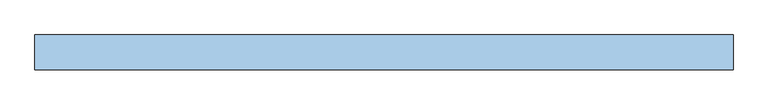
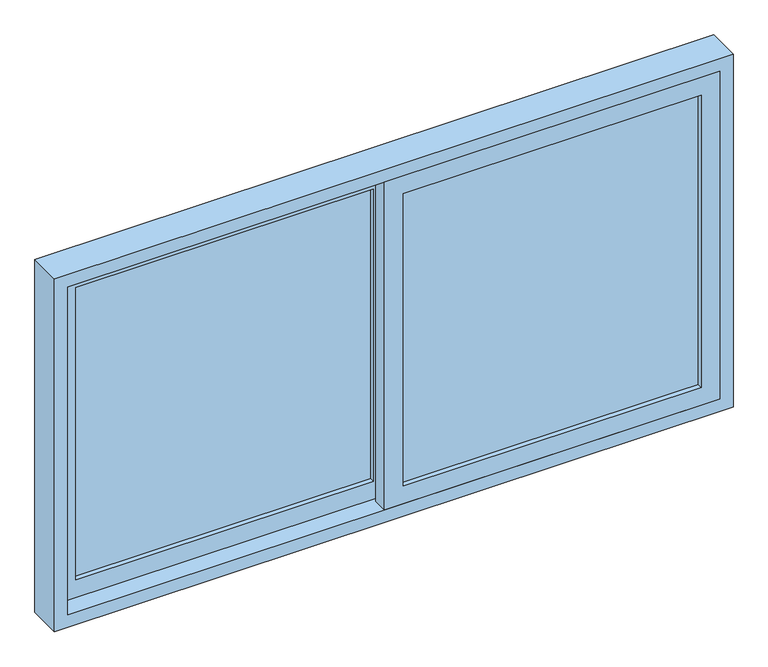
"""IFC4 building model written with IfcOpenShell, lengths in millimetres: window geometry, Janela de correr - 2 Painéis : Janela de correr - 2 Painéis."""

from ifc_helpers import new_model, si_unit, frame, origin, place, context, project, spatial, polyline, outline, extrude, source, transform, mapped, element, save


def window_c87cad41(model_context):
    return source(origin(), model_context, "Body", "SweptSolid", [
        extrude(outline(polyline([(1605.0, -25.0), (685.0, -25.0), (685.0, 865.0), (1605.0, 865.0), (1605.0, -25.0)]), holes=[polyline([(735.0, 25.0), (1555.0, 25.0), (1555.0, 815.0), (735.0, 815.0), (735.0, 25.0)])]), frame((0.0, -20.0, 0.0), z_axis=(0.0, 1.0, 0.0), x_axis=(0.0, 0.0, 1.0)), (0.0, 0.0, 1.0), 40.0),
        extrude(outline(polyline([(685.0, 25.0), (1605.0, 25.0), (1605.0, -865.0), (685.0, -865.0), (685.0, 25.0)]), holes=[polyline([(1555.0, -25.0), (735.0, -25.0), (735.0, -815.0), (1555.0, -815.0), (1555.0, -25.0)])]), frame((0.0, 30.0, 0.0), z_axis=(0.0, 1.0, 0.0), x_axis=(0.0, 0.0, 1.0)), (0.0, 0.0, 1.0), 40.0),
        extrude(outline(polyline([(650.0, 900.0), (1640.0, 900.0), (1640.0, -900.0), (650.0, -900.0), (650.0, 900.0)]), holes=[polyline([(1605.0, 865.0), (685.0, 865.0), (685.0, -865.0), (1605.0, -865.0), (1605.0, 865.0)])]), frame((0.0, -20.0, 0.0), z_axis=(0.0, 1.0, 0.0), x_axis=(0.0, 0.0, 1.0)), (0.0, 0.0, 1.0), 90.0),
        extrude(outline(polyline([(25.0, -7.0), (25.0, 7.0), (815.0, 7.0), (815.0, -7.0), (25.0, -7.0)])), frame((0.0, 0.0, 735.0), z_axis=(0.0, 0.0, 1.0), x_axis=(1.0, 0.0, 0.0)), (0.0, 0.0, 1.0), 820.0),
        extrude(outline(polyline([(-815.0, 43.0), (-815.0, 57.0), (-25.0, 57.0), (-25.0, 43.0), (-815.0, 43.0)])), frame((0.0, 0.0, 735.0), z_axis=(0.0, 0.0, 1.0), x_axis=(1.0, 0.0, 0.0)), (0.0, 0.0, 1.0), 820.0),
    ])


if __name__ == "__main__":
    model = new_model("IFC4")
    model_context = context("Model", 3, world=origin())
    ifc_project = project(units=[si_unit("LENGTHUNIT", "METRE", prefix="MILLI")], contexts=[model_context])
    site = spatial("IfcSite", under=ifc_project)
    building = spatial("IfcBuilding", under=site)
    placement = place(None, origin())
    window_shape = window_c87cad41(model_context)
    element("IfcWindow", 1, ObjectType="Janela de correr - 2 Painéis : Janela de correr - 2 Painéis", at=placement, inside=building, context=model_context, shape_type="MappedRepresentation", body=[
        mapped(window_shape, transform((0.0, 0.0, 0.0), x_axis=(1.0, 0.0, 0.0), y_axis=(0.0, 1.0, 0.0), z_axis=(0.0, 0.0, 1.0))),
    ])
    save(model, "model.ifc")

# Revit data of these elements
# Type "Janela de correr - 2 Painéis : Janela de correr - 2 Painéis"
#   Type Mark = "EF27"
#   Construction Type Id = "GSP4R"
#   Analytic Construction = "Vidraça única Pilkington 1/8 pol"
#   Visual Light Transmittance = 0.9
#   Solar Heat Gain Coefficient = 0.78
#   Rough Width = 1.800 m
#   Rough Height = 0.990 m
#   Largura da moldura do painel = 0.050 m
#   Espessura da moldura do painel = 0.040 m
#   Height = 0.990 m
#   Heat Transfer Coefficient (U) = 3.6886 W/(m²·K)
#   Largura da estrutura = 0.035 m
#   Espessura da moldura = 0.090 m
#   Altura-padrão do peitoril = 0.650 m
#   Width = 1.800 m
#   Define Thermal Properties by = 1
#   Vidro = none
#   Material da moldura = none
#   Wall Closure = (empty or 0)
# Element 1 (IfcWindow, "Janela de correr - 2 Painéis : Janela de correr - 2 Painéis")
#   Materials on its faces: "Glass"
# Materials
#   "Glass": class "Glass", colour RGB 0 128 192, transparency 0.75, Description = "Soda Lime Glass", Cost = 0
